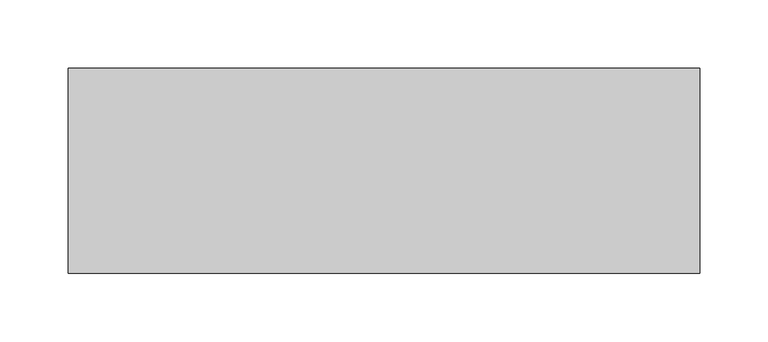
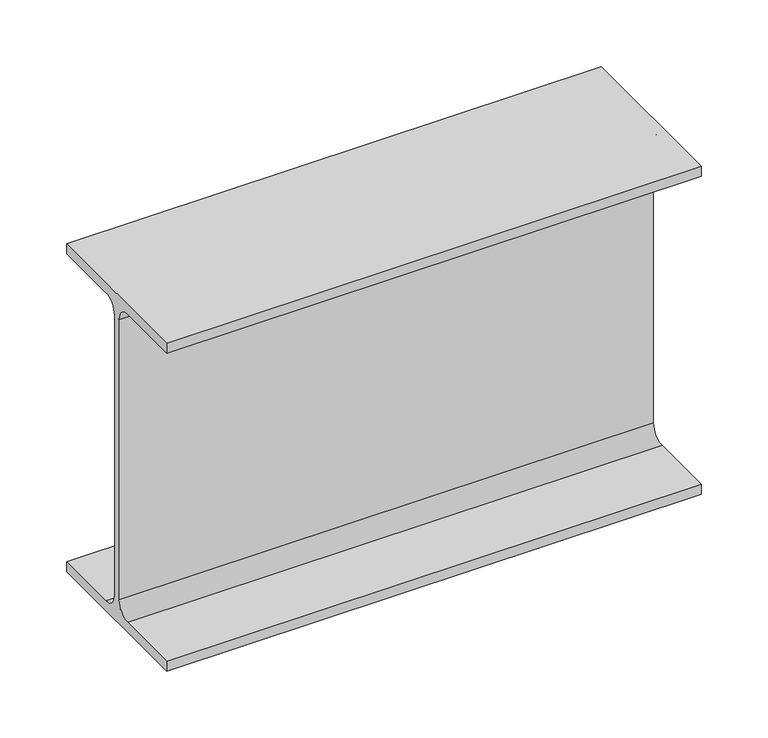
"""IFC4 building model written with IfcOpenShell, lengths in millimetres: beam geometry, 0912_Steel Framing_H-KSD3502 : H_SB_ASB_H-300x150x6.5x9."""

from ifc_helpers import new_model, si_unit, point, frame, frame_2d, origin, place, context, project, spatial, polyline, circle_curve, trimmed, segment, composite_curve, outline, extrude, source, transform, mapped, element, save


def beam_ae00e773(model_context):
    return source(origin(), model_context, "Body", "SweptSolid", [
        extrude(outline(composite_curve([segment(polyline([(75.0, -141.0), (75.0, -150.0), (-75.0, -150.0), (-75.0, -141.0), (-16.25, -141.0)]), True, "CONTINUOUS"), segment(trimmed(circle_curve(frame_2d((-16.25, -128.0)), 13.0), [point((-16.25, -141.0))], [point((-3.25, -128.0))], True, "CARTESIAN"), True, "CONTINUOUS"), segment(polyline([(-3.25, -128.0), (-3.25, 128.0)]), True, "CONTINUOUS"), segment(trimmed(circle_curve(frame_2d((-16.25, 128.0)), 13.0), [point((-3.25, 128.0))], [point((-16.25, 141.0))], True, "CARTESIAN"), True, "CONTINUOUS"), segment(polyline([(-16.25, 141.0), (-75.0, 141.0), (-75.0, 150.0), (75.0, 150.0), (75.0, 141.0), (16.25, 141.0)]), True, "CONTINUOUS"), segment(trimmed(circle_curve(frame_2d((16.25, 128.0)), 13.0), [point((16.25, 141.0))], [point((3.25, 128.0))], True, "CARTESIAN"), True, "CONTINUOUS"), segment(polyline([(3.25, 128.0), (3.25, -128.0)]), True, "CONTINUOUS"), segment(trimmed(circle_curve(frame_2d((16.25, -128.0)), 13.0), [point((3.25, -128.0))], [point((16.25, -141.0))], True, "CARTESIAN"), True, "CONTINUOUS"), segment(polyline([(16.25, -141.0), (75.0, -141.0)]), True, "CONTINUOUS")], self_intersect=False)), frame((-300.0, 0.0, 0.0), z_axis=(1.0, 0.0, 0.0), x_axis=(0.0, 1.0, 0.0)), (0.0, 0.0, 1.0), 462.3),
    ])


if __name__ == "__main__":
    model = new_model("IFC4")
    model_context = context("Model", 3, world=origin())
    ifc_project = project(units=[si_unit("LENGTHUNIT", "METRE", prefix="MILLI")], contexts=[model_context])
    site = spatial("IfcSite", under=ifc_project)
    building = spatial("IfcBuilding", under=site)
    placement = place(None, origin())
    beam_shape = beam_ae00e773(model_context)
    element("IfcBeam", 1, ObjectType="0912_Steel Framing_H-KSD3502 : H_SB_ASB_H-300x150x6.5x9", at=placement, inside=building, context=model_context, shape_type="MappedRepresentation", body=[
        mapped(beam_shape, transform((0.0, 0.0, 0.0), x_axis=(1.0, 0.0, 0.0), y_axis=(0.0, 1.0, 0.0), z_axis=(0.0, 0.0, 1.0))),
    ])
    save(model, "model.ifc")

# Revit data of these elements
# Type "0912_Steel Framing_H-KSD3502 : H_SB_ASB_H-300x150x6.5x9"
#   H_WM Code_1 = "S01AA002-00001 | Main Steel Structure Fabrication Work | Shelter/Building | Medium Steel - Standard (90KG/M>Weight≥30KG/M) | Material: (   )"
#   H_WM Code_2 = "S03AA028-00001 | Main Steel Structure Erection Work | Shelter/Building | Medium Steel (90KG/M>Weight≥30KG/M) | Material: (   )"
#   H_WM Code_3 = "S01AA010-00001 | Main Steel Structure Fabrication Work | Shelter/Building | Steel Painting/Coating | for Non-Fireproofed Steel Surface, Surface Preparation, Primer, Second & Final Coat | Material: (   )"
#   H_Q'ty Cal Type Tag = "SB-Q2"
#   Width = 15.0 cm
#   Web Thickness = 0.65 cm
#   Web Fillet = 1.3 cm
#   Warping Constant = 107000.0 cm⁶
#   W = 0
#   Torsional Moment of Inertia = 9.9539 cm⁴
#   Section Area = 46.78 cm²
#   Plastic Modulus weak axis = 105.0 cm³
#   Plastic Modulus strong axis = 542.0 cm³
#   Perimeter = 1.17 m²/m
#   Nominal Weight = 36.70 kgf/m
#   Moment of Inertia weak axis = 508.00 cm⁴
#   Moment of Inertia strong axis = 7210.00 cm⁴
#   Height = 30.0 cm
#   Flange Thickness = 0.9 cm
#   Elastic Modulus weak axis = 67.7 cm³
#   Elastic Modulus strong axis = 481.0 cm³
#   Centroid Vertical = 15.0 cm
#   Centroid Horizontal = 7.5 cm
#   Ix = 72100000
#   Length [instance default] = 1.5240 m
#   Zx = 542000
#   b = 0.1500 m
#   h = 0.3000 m
#   r = 0.0130 m
#   s = 0.0065 m
#   t = 0.0090 m
#   A = 0.004678 m²
#   Structural Material [instance default] = Steel, 45-345
#   Assembly Code = ""
# Element 1 (IfcBeam, "0912_Steel Framing_H-KSD3502 : H_SB_ASB_H-300x150x6.5x9")
#   Structural Material = none
# Materials
#   "Steel, 45-345": class "Metal", colour RGB 189 187 185, transparency 0, Description = "Steel 345 MPa", Cost = 0
